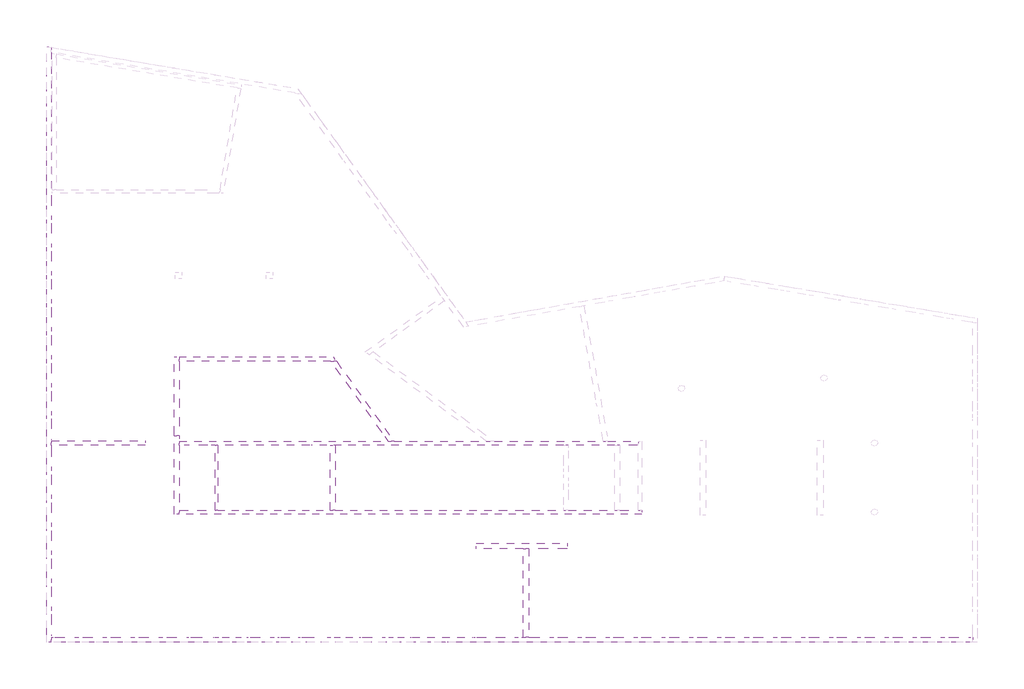
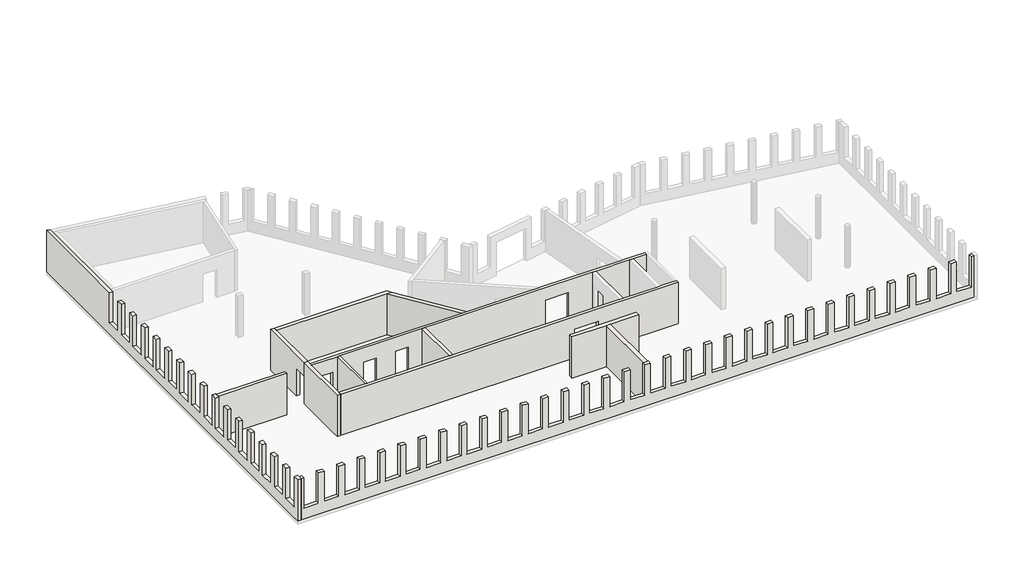
# One storey, part 1 of 2: 13 walls.
"""IFC4 building model written with IfcOpenShell, lengths in millimetres."""

from ifc_helpers import new_model, si_unit, frame, origin, place, context, project, spatial, polyline, outline, extrude, faceted_brep, element, save

model = new_model("IFC4")

# Units and contexts
model_context = context("Model", 3, world=origin())
ifc_project = project(units=[si_unit("LENGTHUNIT", "METRE", prefix="MILLI")], contexts=[model_context])

# Site, building, storey
site = spatial("IfcSite", under=ifc_project)
building = spatial("IfcBuilding", under=site)
storey = spatial("IfcBuildingStorey", under=building, Name="01_UG_OKFB_-4,20", Elevation=-4200.0)

# Walls
placement = place(None, origin())
element("IfcWall", 1, ObjectType="5dki Lochfassade 26cm C30/37", at=placement, inside=storey, context=model_context, shape_type="Brep", body=[
    faceted_brep([(130.0010047, 22777.9895381, 710.0), (130.0010047, 22777.9895381, 3060.0), (130.0010047, 22357.0124158, 3060.0), (130.0010047, 22357.0124158, 710.0), (130.0010047, 21277.0124158, 710.0), (130.0010047, 21277.0124158, 3060.0), (130.0010047, 20857.0124158, 3060.0), (130.0010047, 20857.0124158, 710.0), (130.0010047, 19777.0124158, 710.0), (130.0010047, 19777.0124158, 3060.0), (130.0010047, 19357.0124158, 3060.0), (130.0010047, 19357.0124158, 710.0), (130.0010047, 18277.0124158, 710.0), (130.0010047, 18277.0124158, 3060.0), (130.0010047, 17857.0124158, 3060.0), (130.0010047, 17857.0124158, 710.0), (130.0010047, 16777.0124158, 710.0), (130.0010047, 16777.0124158, 3060.0), (130.0010047, 16357.0124158, 3060.0), (130.0010047, 16357.0124158, 710.0), (130.0010047, 15277.0124158, 710.0), (130.0010047, 15277.0124158, 3060.0), (130.0010047, 14857.0124158, 3060.0), (130.0010047, 14857.0124158, 710.0), (130.0010047, 13777.0124158, 710.0), (130.0010047, 13777.0124158, 3060.0), (130.0010047, 13357.0124158, 3060.0), (130.0010047, 13357.0124158, 710.0), (130.0010047, 12277.0124158, 710.0), (130.0010047, 12277.0124158, 3060.0), (130.0010047, 11857.0124158, 3060.0), (130.0010047, 11857.0124158, 710.0), (130.0010047, 10777.0124158, 710.0), (130.0010047, 10777.0124158, 3060.0), (130.0010047, 10692.0124295, 3060.0), (130.0010047, 10442.0124295, 3060.0), (130.0010047, 10357.0124158, 3060.0), (130.0010047, 10357.0124158, 710.0), (130.0010047, 9277.0124158, 710.0), (130.0010047, 9277.0124158, 3060.0), (130.0010047, 8857.0124158, 3060.0), (130.0010047, 8857.0124158, 710.0), (130.0010047, 7777.0124158, 710.0), (130.0010047, 7777.0124158, 3060.0), (130.0010047, 7357.0124158, 3060.0), (130.0010047, 7357.0124158, 710.0), (130.0010047, 6277.0124158, 710.0), (130.0010047, 6277.0124158, 3060.0), (130.0010047, 5857.0124158, 3060.0), (130.0010047, 5857.0124158, 710.0), (130.0010047, 4777.0124158, 710.0), (130.0010047, 4777.0124158, 3060.0), (130.0010047, 4357.0124158, 3060.0), (130.0010047, 4357.0124158, 710.0), (130.0010047, 3277.0124158, 710.0), (130.0010047, 3277.0124158, 3060.0), (130.0010047, 2857.0124158, 3060.0), (130.0010047, 2857.0124158, 710.0), (130.0010047, 1777.0124158, 710.0), (130.0010047, 1777.0124158, 3060.0), (130.0010047, 1357.0124158, 3060.0), (130.0010047, 1357.0124158, 710.0), (130.0010047, 277.0124158, 710.0), (130.0010047, 277.0124158, 3060.0), (130.0010047, 130.000972, 3060.0), (130.0010047, -129.999028, 3060.0), (130.0010047, -129.999028, -150.0), (130.0010047, 130.000972, -150.0), (130.0010047, 10442.0124295, -150.0), (130.0010047, 10692.0124295, -150.0), (130.0010047, 31548.6978518, -150.0), (130.0010047, 31812.2980067, -150.0), (130.0010047, 31812.2980067, 3060.0), (130.0010047, 31548.6978518, 3060.0), (130.0010047, 23857.9895381, 3060.0), (130.0010047, 23857.9895381, 710.0), (-129.9989953, 22357.0124158, 3060.0), (-129.9989953, 22777.9895381, 3060.0), (-129.9989953, 22777.9895381, 710.0), (-129.9989953, 23857.9895381, 710.0), (-129.9989953, 23857.9895381, 3060.0), (-129.9989953, 31855.7150729, 3060.0), (-129.9989953, 31855.7150729, -150.0), (-129.9989953, -129.9990284, -150.0), (-129.9989953, -129.9990284, 3060.0), (-129.9989953, 277.0124158, 3060.0), (-129.9989953, 277.0124158, 710.0), (-129.9989953, 1357.0124158, 710.0), (-129.9989953, 1357.0124158, 3060.0), (-129.9989953, 1777.0124158, 3060.0), (-129.9989953, 1777.0124158, 710.0), (-129.9989953, 2857.0124158, 710.0), (-129.9989953, 2857.0124158, 3060.0), (-129.9989953, 3277.0124158, 3060.0), (-129.9989953, 3277.0124158, 710.0), (-129.9989953, 4357.0124158, 710.0), (-129.9989953, 4357.0124158, 3060.0), (-129.9989953, 4777.0124158, 3060.0), (-129.9989953, 4777.0124158, 710.0), (-129.9989953, 5857.0124158, 710.0), (-129.9989953, 5857.0124158, 3060.0), (-129.9989953, 6277.0124158, 3060.0), (-129.9989953, 6277.0124158, 710.0), (-129.9989953, 7357.0124158, 710.0), (-129.9989953, 7357.0124158, 3060.0), (-129.9989953, 7777.0124158, 3060.0), (-129.9989953, 7777.0124158, 710.0), (-129.9989953, 8857.0124158, 710.0), (-129.9989953, 8857.0124158, 3060.0), (-129.9989953, 9277.0124158, 3060.0), (-129.9989953, 9277.0124158, 710.0), (-129.9989953, 10357.0124158, 710.0), (-129.9989953, 10357.0124158, 3060.0), (-129.9989953, 10777.0124158, 3060.0), (-129.9989953, 10777.0124158, 710.0), (-129.9989953, 11857.0124158, 710.0), (-129.9989953, 11857.0124158, 3060.0), (-129.9989953, 12277.0124158, 3060.0), (-129.9989953, 12277.0124158, 710.0), (-129.9989953, 13357.0124158, 710.0), (-129.9989953, 13357.0124158, 3060.0), (-129.9989953, 13777.0124158, 3060.0), (-129.9989953, 13777.0124158, 710.0), (-129.9989953, 14857.0124158, 710.0), (-129.9989953, 14857.0124158, 3060.0), (-129.9989953, 15277.0124158, 3060.0), (-129.9989953, 15277.0124158, 710.0), (-129.9989953, 16357.0124158, 710.0), (-129.9989953, 16357.0124158, 3060.0), (-129.9989953, 16777.0124158, 3060.0), (-129.9989953, 16777.0124158, 710.0), (-129.9989953, 17857.0124158, 710.0), (-129.9989953, 17857.0124158, 3060.0), (-129.9989953, 18277.0124158, 3060.0), (-129.9989953, 18277.0124158, 710.0), (-129.9989953, 19357.0124158, 710.0), (-129.9989953, 19357.0124158, 3060.0), (-129.9989953, 19777.0124158, 3060.0), (-129.9989953, 19777.0124158, 710.0), (-129.9989953, 20857.0124158, 710.0), (-129.9989953, 20857.0124158, 3060.0), (-129.9989953, 21277.0124158, 3060.0), (-129.9989953, 21277.0124158, 710.0), (-129.9989953, 22357.0124158, 710.0)], [[[0, 1, 2, 3, 4, 5, 6, 7, 8, 9, 10, 11, 12, 13, 14, 15, 16, 17, 18, 19, 20, 21, 22, 23, 24, 25, 26, 27, 28, 29, 30, 31, 32, 33, 34, 35, 36, 37, 38, 39, 40, 41, 42, 43, 44, 45, 46, 47, 48, 49, 50, 51, 52, 53, 54, 55, 56, 57, 58, 59, 60, 61, 62, 63, 64, 65, 66, 67, 68, 69, 70, 71, 72, 73, 74, 75]], [[76, 77, 78, 79, 80, 81, 82, 83, 84, 85, 86, 87, 88, 89, 90, 91, 92, 93, 94, 95, 96, 97, 98, 99, 100, 101, 102, 103, 104, 105, 106, 107, 108, 109, 110, 111, 112, 113, 114, 115, 116, 117, 118, 119, 120, 121, 122, 123, 124, 125, 126, 127, 128, 129, 130, 131, 132, 133, 134, 135, 136, 137, 138, 139, 140, 141, 142, 143]], [[71, 70, 69, 68, 67, 66, 83, 82]], [[84, 65, 64, 63, 85]], [[60, 59, 89, 88]], [[56, 55, 93, 92]], [[52, 51, 97, 96]], [[48, 47, 101, 100]], [[44, 43, 105, 104]], [[40, 39, 109, 108]], [[36, 35, 34, 33, 113, 112]], [[30, 29, 117, 116]], [[26, 25, 121, 120]], [[22, 21, 125, 124]], [[18, 17, 129, 128]], [[14, 13, 133, 132]], [[10, 9, 137, 136]], [[6, 5, 141, 140]], [[2, 1, 77, 76]], [[74, 73, 72, 81, 80]], [[72, 71, 82, 81]], [[66, 65, 84, 83]], [[87, 61, 60, 88]], [[62, 86, 85, 63]], [[61, 87, 86, 62]], [[92, 91, 57, 56]], [[90, 89, 59, 58]], [[91, 90, 58, 57]], [[96, 95, 53, 52]], [[94, 93, 55, 54]], [[95, 94, 54, 53]], [[100, 99, 49, 48]], [[98, 97, 51, 50]], [[99, 98, 50, 49]], [[104, 103, 45, 44]], [[102, 101, 47, 46]], [[103, 102, 46, 45]], [[108, 107, 41, 40]], [[106, 105, 43, 42]], [[107, 106, 42, 41]], [[112, 111, 37, 36]], [[110, 109, 39, 38]], [[111, 110, 38, 37]], [[116, 115, 31, 30]], [[114, 113, 33, 32]], [[115, 114, 32, 31]], [[120, 119, 27, 26]], [[118, 117, 29, 28]], [[119, 118, 28, 27]], [[124, 123, 23, 22]], [[122, 121, 25, 24]], [[123, 122, 24, 23]], [[128, 127, 19, 18]], [[126, 125, 21, 20]], [[127, 126, 20, 19]], [[132, 131, 15, 14]], [[130, 129, 17, 16]], [[131, 130, 16, 15]], [[136, 135, 11, 10]], [[134, 133, 13, 12]], [[135, 134, 12, 11]], [[140, 139, 7, 6]], [[138, 137, 9, 8]], [[139, 138, 8, 7]], [[76, 143, 3, 2]], [[142, 141, 5, 4]], [[143, 142, 4, 3]], [[80, 79, 75, 74]], [[78, 77, 1, 0]], [[79, 78, 0, 75]]]),
])
element("IfcWall", 2, ObjectType="5dki Lochfassade 26cm C30/37", at=placement, inside=storey, context=model_context, shape_type="Brep", body=[
    faceted_brep([(49396.9999991, 130.0010483, 710.0), (49396.9999991, 130.0010483, 3060.0), (49603.9991101, 130.0010486, 3060.0), (49603.9991101, 130.0010486, -150.0), (25766.9999915, 130.0010117, -150.0), (25466.9999915, 130.0010113, -150.0), (130.0010047, 130.000972, -150.0), (130.0010047, 130.000972, 3060.0), (317.0000012, 130.0009723, 3060.0), (316.999997, 130.0009723, 710.0), (1397.0000012, 130.000974, 710.0), (1397.0000069, 130.000974, 3060.0), (1816.9999991, 130.0009747, 3060.0), (1817.0000028, 130.0009747, 710.0), (2896.9999991, 130.0009763, 710.0), (2897.0000017, 130.0009763, 3060.0), (3316.9999991, 130.000977, 3060.0), (3316.9999977, 130.000977, 710.0), (4396.9999991, 130.0009787, 710.0), (4396.9999966, 130.0009787, 3060.0), (4816.9999991, 130.0009793, 3060.0), (4816.9999991, 130.0009793, 710.0), (5896.9999991, 130.000981, 710.0), (5896.9999991, 130.000981, 3060.0), (6316.9999991, 130.0009816, 3060.0), (6316.9999991, 130.0009816, 710.0), (7396.9999991, 130.0009833, 710.0), (7396.9999991, 130.0009833, 3060.0), (7816.9999991, 130.0009839, 3060.0), (7816.9999991, 130.0009839, 710.0), (8896.9999991, 130.0009856, 710.0), (8896.9999991, 130.0009856, 3060.0), (9316.9999991, 130.0009863, 3060.0), (9316.9999991, 130.0009863, 710.0), (10396.9999991, 130.0009879, 710.0), (10396.9999991, 130.0009879, 3060.0), (10816.9999991, 130.0009886, 3060.0), (10816.9999991, 130.0009886, 710.0), (11896.9999991, 130.0009903, 710.0), (11896.9999991, 130.0009903, 3060.0), (12316.9999991, 130.0009909, 3060.0), (12316.9999991, 130.0009909, 710.0), (13396.9999991, 130.0009926, 710.0), (13396.9999991, 130.0009926, 3060.0), (13816.9999991, 130.0009932, 3060.0), (13816.9999991, 130.0009932, 710.0), (14896.9999991, 130.0009949, 710.0), (14896.9999991, 130.0009949, 3060.0), (15316.9999991, 130.0009956, 3060.0), (15316.9999991, 130.0009956, 710.0), (16396.9999991, 130.0009972, 710.0), (16396.9999991, 130.0009972, 3060.0), (16816.9999991, 130.0009979, 3060.0), (16816.9999991, 130.0009979, 710.0), (17896.9999991, 130.0009996, 710.0), (17896.9999991, 130.0009996, 3060.0), (18316.9999991, 130.0010002, 3060.0), (18316.9999991, 130.0010002, 710.0), (19396.9999991, 130.0010019, 710.0), (19396.9999991, 130.0010019, 3060.0), (19816.9999991, 130.0010025, 3060.0), (19816.9999991, 130.0010025, 710.0), (20896.9999991, 130.0010042, 710.0), (20896.9999991, 130.0010042, 3060.0), (21316.9999991, 130.0010048, 3060.0), (21316.9999991, 130.0010048, 710.0), (22396.9999991, 130.0010065, 710.0), (22396.9999991, 130.0010065, 3060.0), (22816.9999991, 130.0010072, 3060.0), (22816.9999991, 130.0010072, 710.0), (23896.9999991, 130.0010088, 710.0), (23896.9999991, 130.0010088, 3060.0), (24316.9999991, 130.0010095, 3060.0), (24316.9999991, 130.0010095, 710.0), (25396.9999991, 130.0010112, 710.0), (25396.9999991, 130.0010112, 3060.0), (25466.9999915, 130.0010113, 3060.0), (25766.9999915, 130.0010117, 3060.0), (25816.9999991, 130.0010118, 3060.0), (25816.9999991, 130.0010118, 710.0), (26896.9999991, 130.0010135, 710.0), (26896.9999991, 130.0010135, 3060.0), (27316.9999991, 130.0010141, 3060.0), (27316.9999991, 130.0010141, 710.0), (28396.9999991, 130.0010158, 710.0), (28396.9999991, 130.0010158, 3060.0), (28816.9999991, 130.0010165, 3060.0), (28816.9999991, 130.0010165, 710.0), (29896.9999991, 130.0010181, 710.0), (29896.9999991, 130.0010181, 3060.0), (30316.9999991, 130.0010188, 3060.0), (30316.9999991, 130.0010188, 710.0), (31396.9999991, 130.0010205, 710.0), (31396.9999991, 130.0010205, 3060.0), (31816.9999991, 130.0010211, 3060.0), (31816.9999991, 130.0010211, 710.0), (32896.9999991, 130.0010228, 710.0), (32896.9999991, 130.0010228, 3060.0), (33316.9999991, 130.0010234, 3060.0), (33316.9999991, 130.0010234, 710.0), (34396.9999991, 130.0010251, 710.0), (34396.9999991, 130.0010251, 3060.0), (34816.9999991, 130.0010258, 3060.0), (34816.9999991, 130.0010258, 710.0), (35896.9999991, 130.0010274, 710.0), (35896.9999991, 130.0010274, 3060.0), (36316.9999991, 130.0010281, 3060.0), (36316.9999991, 130.0010281, 710.0), (37396.9999991, 130.0010297, 710.0), (37396.9999991, 130.0010297, 3060.0), (37816.9999991, 130.0010304, 3060.0), (37816.9999991, 130.0010304, 710.0), (38896.9999991, 130.0010321, 710.0), (38896.9999991, 130.0010321, 3060.0), (39316.9999991, 130.0010327, 3060.0), (39316.9999991, 130.0010327, 710.0), (40396.9999991, 130.0010344, 710.0), (40396.9999991, 130.0010344, 3060.0), (40816.9999991, 130.001035, 3060.0), (40816.9999991, 130.001035, 710.0), (41896.9999991, 130.0010367, 710.0), (41896.9999991, 130.0010367, 3060.0), (42316.9999991, 130.0010374, 3060.0), (42316.9999991, 130.0010374, 710.0), (43396.9999991, 130.001039, 710.0), (43396.9999991, 130.001039, 3060.0), (43816.9999991, 130.0010397, 3060.0), (43816.9999991, 130.0010397, 710.0), (44896.9999991, 130.0010414, 710.0), (44896.9999991, 130.0010414, 3060.0), (45316.9999991, 130.001042, 3060.0), (45316.9999991, 130.001042, 710.0), (46396.9999991, 130.0010437, 710.0), (46396.9999991, 130.0010437, 3060.0), (46816.9999991, 130.0010443, 3060.0), (46816.9999991, 130.0010443, 710.0), (47896.9999991, 130.001046, 710.0), (47896.9999991, 130.001046, 3060.0), (48316.9999991, 130.0010467, 3060.0), (48316.9999991, 130.0010467, 710.0), (49603.9991105, -129.9989514, 3060.0), (49396.9999995, -129.9989517, 3060.0), (49396.9999995, -129.9989517, 710.0), (48316.9999995, -129.9989533, 710.0), (48316.9999995, -129.9989533, 3060.0), (47896.9999995, -129.998954, 3060.0), (47896.9999995, -129.998954, 710.0), (46816.9999995, -129.9989557, 710.0), (46816.9999995, -129.9989557, 3060.0), (46396.9999995, -129.9989563, 3060.0), (46396.9999995, -129.9989563, 710.0), (45316.9999995, -129.998958, 710.0), (45316.9999995, -129.998958, 3060.0), (44896.9999995, -129.9989586, 3060.0), (44896.9999995, -129.9989586, 710.0), (43816.9999995, -129.9989603, 710.0), (43816.9999995, -129.9989603, 3060.0), (43396.9999995, -129.998961, 3060.0), (43396.9999995, -129.998961, 710.0), (42316.9999995, -129.9989626, 710.0), (42316.9999995, -129.9989626, 3060.0), (41896.9999995, -129.9989633, 3060.0), (41896.9999995, -129.9989633, 710.0), (40816.9999995, -129.998965, 710.0), (40816.9999995, -129.998965, 3060.0), (40396.9999995, -129.9989656, 3060.0), (40396.9999995, -129.9989656, 710.0), (39316.9999995, -129.9989673, 710.0), (39316.9999995, -129.9989673, 3060.0), (38896.9999995, -129.9989679, 3060.0), (38896.9999995, -129.9989679, 710.0), (37816.9999995, -129.9989696, 710.0), (37816.9999995, -129.9989696, 3060.0), (37396.9999995, -129.9989703, 3060.0), (37396.9999995, -129.9989703, 710.0), (36316.9999995, -129.9989719, 710.0), (36316.9999995, -129.9989719, 3060.0), (35896.9999995, -129.9989726, 3060.0), (35896.9999995, -129.9989726, 710.0), (34816.9999995, -129.9989742, 710.0), (34816.9999995, -129.9989742, 3060.0), (34396.9999995, -129.9989749, 3060.0), (34396.9999995, -129.9989749, 710.0), (33316.9999995, -129.9989766, 710.0), (33316.9999995, -129.9989766, 3060.0), (32896.9999995, -129.9989772, 3060.0), (32896.9999995, -129.9989772, 710.0), (31816.9999995, -129.9989789, 710.0), (31816.9999995, -129.9989789, 3060.0), (31396.9999995, -129.9989795, 3060.0), (31396.9999995, -129.9989795, 710.0), (30316.9999995, -129.9989812, 710.0), (30316.9999995, -129.9989812, 3060.0), (29896.9999995, -129.9989819, 3060.0), (29896.9999995, -129.9989819, 710.0), (28816.9999995, -129.9989835, 710.0), (28816.9999995, -129.9989835, 3060.0), (28396.9999995, -129.9989842, 3060.0), (28396.9999995, -129.9989842, 710.0), (27316.9999995, -129.9989859, 710.0), (27316.9999995, -129.9989859, 3060.0), (26896.9999995, -129.9989865, 3060.0), (26896.9999995, -129.9989865, 710.0), (25816.9999995, -129.9989882, 710.0), (25816.9999995, -129.9989882, 3060.0), (25396.9999995, -129.9989888, 3060.0), (25396.9999995, -129.9989888, 710.0), (24316.9999995, -129.9989905, 710.0), (24316.9999995, -129.9989905, 3060.0), (23896.9999995, -129.9989912, 3060.0), (23896.9999995, -129.9989912, 710.0), (22816.9999995, -129.9989928, 710.0), (22816.9999995, -129.9989928, 3060.0), (22396.9999995, -129.9989935, 3060.0), (22396.9999995, -129.9989935, 710.0), (21316.9999995, -129.9989952, 710.0), (21316.9999995, -129.9989952, 3060.0), (20896.9999995, -129.9989958, 3060.0), (20896.9999995, -129.9989958, 710.0), (19816.9999995, -129.9989975, 710.0), (19816.9999995, -129.9989975, 3060.0), (19396.9999995, -129.9989981, 3060.0), (19396.9999995, -129.9989981, 710.0), (18316.9999995, -129.9989998, 710.0), (18316.9999995, -129.9989998, 3060.0), (17896.9999995, -129.9990004, 3060.0), (17896.9999995, -129.9990004, 710.0), (16816.9999995, -129.9990021, 710.0), (16816.9999995, -129.9990021, 3060.0), (16396.9999995, -129.9990028, 3060.0), (16396.9999995, -129.9990028, 710.0), (15316.9999995, -129.9990044, 710.0), (15316.9999995, -129.9990044, 3060.0), (14896.9999995, -129.9990051, 3060.0), (14896.9999995, -129.9990051, 710.0), (13816.9999995, -129.9990068, 710.0), (13816.9999995, -129.9990068, 3060.0), (13396.9999995, -129.9990074, 3060.0), (13396.9999995, -129.9990074, 710.0), (12316.9999995, -129.9990091, 710.0), (12316.9999995, -129.9990091, 3060.0), (11896.9999995, -129.9990097, 3060.0), (11896.9999995, -129.9990097, 710.0), (10816.9999995, -129.9990114, 710.0), (10816.9999995, -129.9990114, 3060.0), (10396.9999995, -129.9990121, 3060.0), (10396.9999995, -129.9990121, 710.0), (9316.9999995, -129.9990137, 710.0), (9316.9999995, -129.9990137, 3060.0), (8896.9999995, -129.9990144, 3060.0), (8896.9999995, -129.9990144, 710.0), (7816.9999995, -129.9990161, 710.0), (7816.9999995, -129.9990161, 3060.0), (7396.9999995, -129.9990167, 3060.0), (7396.9999995, -129.9990167, 710.0), (6316.9999995, -129.9990184, 710.0), (6316.9999995, -129.9990184, 3060.0), (5896.9999995, -129.999019, 3060.0), (5896.9999995, -129.999019, 710.0), (4816.9999995, -129.9990207, 710.0), (4816.9999995, -129.9990207, 3060.0), (4396.9999995, -129.9990213, 3060.0), (4396.9999966, -129.9990213, 710.0), (3316.9999995, -129.999023, 710.0), (3316.9999977, -129.999023, 3060.0), (2896.9999995, -129.9990237, 3060.0), (2897.0000017, -129.9990237, 710.0), (1816.9999995, -129.9990253, 710.0), (1817.0000028, -129.9990253, 3060.0), (1397.0000016, -129.999026, 3060.0), (1397.0000069, -129.999026, 710.0), (317.0000016, -129.9990277, 710.0), (316.999997, -129.9990277, 3060.0), (130.0010047, -129.999028, 3060.0), (130.0010047, -129.999028, -150.0), (49603.9991105, -129.9989514, -150.0)], [[[0, 1, 2, 3, 4, 5, 6, 7, 8, 9, 10, 11, 12, 13, 14, 15, 16, 17, 18, 19, 20, 21, 22, 23, 24, 25, 26, 27, 28, 29, 30, 31, 32, 33, 34, 35, 36, 37, 38, 39, 40, 41, 42, 43, 44, 45, 46, 47, 48, 49, 50, 51, 52, 53, 54, 55, 56, 57, 58, 59, 60, 61, 62, 63, 64, 65, 66, 67, 68, 69, 70, 71, 72, 73, 74, 75, 76, 77, 78, 79, 80, 81, 82, 83, 84, 85, 86, 87, 88, 89, 90, 91, 92, 93, 94, 95, 96, 97, 98, 99, 100, 101, 102, 103, 104, 105, 106, 107, 108, 109, 110, 111, 112, 113, 114, 115, 116, 117, 118, 119, 120, 121, 122, 123, 124, 125, 126, 127, 128, 129, 130, 131, 132, 133, 134, 135, 136, 137, 138, 139]], [[140, 141, 142, 143, 144, 145, 146, 147, 148, 149, 150, 151, 152, 153, 154, 155, 156, 157, 158, 159, 160, 161, 162, 163, 164, 165, 166, 167, 168, 169, 170, 171, 172, 173, 174, 175, 176, 177, 178, 179, 180, 181, 182, 183, 184, 185, 186, 187, 188, 189, 190, 191, 192, 193, 194, 195, 196, 197, 198, 199, 200, 201, 202, 203, 204, 205, 206, 207, 208, 209, 210, 211, 212, 213, 214, 215, 216, 217, 218, 219, 220, 221, 222, 223, 224, 225, 226, 227, 228, 229, 230, 231, 232, 233, 234, 235, 236, 237, 238, 239, 240, 241, 242, 243, 244, 245, 246, 247, 248, 249, 250, 251, 252, 253, 254, 255, 256, 257, 258, 259, 260, 261, 262, 263, 264, 265, 266, 267, 268, 269, 270, 271, 272, 273, 274, 275]], [[6, 5, 4, 3, 275, 274]], [[7, 273, 272, 8]], [[15, 265, 264, 16]], [[268, 12, 11, 269]], [[261, 260, 20, 19]], [[257, 256, 24, 23]], [[253, 252, 28, 27]], [[249, 248, 32, 31]], [[245, 244, 36, 35]], [[241, 240, 40, 39]], [[237, 236, 44, 43]], [[233, 232, 48, 47]], [[229, 228, 52, 51]], [[225, 224, 56, 55]], [[221, 220, 60, 59]], [[217, 216, 64, 63]], [[213, 212, 68, 67]], [[209, 208, 72, 71]], [[205, 204, 78, 77, 76, 75]], [[201, 200, 82, 81]], [[197, 196, 86, 85]], [[193, 192, 90, 89]], [[189, 188, 94, 93]], [[185, 184, 98, 97]], [[181, 180, 102, 101]], [[177, 176, 106, 105]], [[173, 172, 110, 109]], [[169, 168, 114, 113]], [[165, 164, 118, 117]], [[161, 160, 122, 121]], [[157, 156, 126, 125]], [[153, 152, 130, 129]], [[149, 148, 134, 133]], [[138, 137, 145, 144]], [[2, 1, 141, 140]], [[7, 6, 274, 273]], [[3, 2, 140, 275]], [[10, 270, 269, 11]], [[271, 9, 8, 272]], [[270, 10, 9, 271]], [[14, 266, 265, 15]], [[267, 13, 12, 268]], [[266, 14, 13, 267]], [[18, 262, 261, 19]], [[263, 17, 16, 264]], [[262, 18, 17, 263]], [[23, 22, 258, 257]], [[21, 20, 260, 259]], [[22, 21, 259, 258]], [[27, 26, 254, 253]], [[25, 24, 256, 255]], [[26, 25, 255, 254]], [[31, 30, 250, 249]], [[29, 28, 252, 251]], [[30, 29, 251, 250]], [[35, 34, 246, 245]], [[33, 32, 248, 247]], [[34, 33, 247, 246]], [[39, 38, 242, 241]], [[37, 36, 244, 243]], [[38, 37, 243, 242]], [[43, 42, 238, 237]], [[41, 40, 240, 239]], [[42, 41, 239, 238]], [[47, 46, 234, 233]], [[45, 44, 236, 235]], [[46, 45, 235, 234]], [[51, 50, 230, 229]], [[49, 48, 232, 231]], [[50, 49, 231, 230]], [[55, 54, 226, 225]], [[53, 52, 228, 227]], [[54, 53, 227, 226]], [[59, 58, 222, 221]], [[57, 56, 224, 223]], [[58, 57, 223, 222]], [[63, 62, 218, 217]], [[61, 60, 220, 219]], [[62, 61, 219, 218]], [[67, 66, 214, 213]], [[65, 64, 216, 215]], [[66, 65, 215, 214]], [[71, 70, 210, 209]], [[69, 68, 212, 211]], [[70, 69, 211, 210]], [[75, 74, 206, 205]], [[73, 72, 208, 207]], [[74, 73, 207, 206]], [[81, 80, 202, 201]], [[79, 78, 204, 203]], [[80, 79, 203, 202]], [[85, 84, 198, 197]], [[83, 82, 200, 199]], [[84, 83, 199, 198]], [[89, 88, 194, 193]], [[87, 86, 196, 195]], [[88, 87, 195, 194]], [[93, 92, 190, 189]], [[91, 90, 192, 191]], [[92, 91, 191, 190]], [[97, 96, 186, 185]], [[95, 94, 188, 187]], [[96, 95, 187, 186]], [[101, 100, 182, 181]], [[99, 98, 184, 183]], [[100, 99, 183, 182]], [[105, 104, 178, 177]], [[103, 102, 180, 179]], [[104, 103, 179, 178]], [[109, 108, 174, 173]], [[107, 106, 176, 175]], [[108, 107, 175, 174]], [[113, 112, 170, 169]], [[111, 110, 172, 171]], [[112, 111, 171, 170]], [[117, 116, 166, 165]], [[115, 114, 168, 167]], [[116, 115, 167, 166]], [[121, 120, 162, 161]], [[119, 118, 164, 163]], [[120, 119, 163, 162]], [[125, 124, 158, 157]], [[123, 122, 160, 159]], [[124, 123, 159, 158]], [[129, 128, 154, 153]], [[127, 126, 156, 155]], [[128, 127, 155, 154]], [[133, 132, 150, 149]], [[131, 130, 152, 151]], [[132, 131, 151, 150]], [[137, 136, 146, 145]], [[135, 134, 148, 147]], [[136, 135, 147, 146]], [[144, 143, 139, 138]], [[142, 141, 1, 0]], [[143, 142, 0, 139]]]),
])
element("IfcWall", 3, ObjectType="5dki STB-Wand Kern 25cm C30/37", at=placement, inside=storey, context=model_context, shape_type="Brep", body=[
    faceted_brep([(6989.9999766, 15192.0124447, 3060.0), (6989.9999766, 14942.0124447, 3060.0), (6989.9999766, 10947.0136187, 3060.0), (6989.9999766, 10947.0136187, 1985.0), (6989.9999766, 11957.013616, 1985.0), (6989.9999766, 11957.013616, -150.0), (6989.9999766, 14942.0124447, -150.0), (6989.9999766, 15192.0124447, -150.0), (6739.9999766, 10947.0136187, 3060.0), (6739.9999766, 15192.0124447, 3060.0), (6739.9999766, 15192.0124447, -150.0), (6739.9999766, 11957.013616, -150.0), (6739.9999766, 11957.013616, 1985.0), (6739.9999766, 10947.0136187, 1985.0)], [[[0, 1, 2, 3, 4, 5, 6, 7]], [[8, 9, 10, 11, 12, 13]], [[10, 7, 6, 5, 11]], [[2, 1, 0, 9, 8]], [[2, 8, 13, 3]], [[0, 7, 10, 9]], [[4, 12, 11, 5]], [[12, 4, 3, 13]]]),
])
element("IfcWall", 4, ObjectType="5dki STB-Wand Kern 25cm C30/37", at=placement, inside=storey, context=model_context, shape_type="Brep", body=[
    faceted_brep([(6989.9999766, 14942.0124447, -150.0), (15141.8279932, 14942.0124447, -150.0), (15449.8792779, 14942.0124447, -150.0), (15449.8792779, 14942.0124447, 3060.0), (15141.8279932, 14942.0124447, 3060.0), (6989.9999766, 14942.0124447, 3060.0), (6989.9999766, 15192.0124447, -150.0), (6989.9999766, 15192.0124447, 3060.0), (15269.8915173, 15192.0124447, 3060.0), (15269.8915173, 15192.0124447, -150.0)], [[[0, 1, 2, 3, 4, 5]], [[6, 7, 8, 9]], [[2, 1, 0, 6, 9]], [[5, 4, 3, 8, 7]], [[0, 5, 7, 6]], [[3, 2, 9, 8]]]),
])
element("IfcWall", 5, ObjectType="5dki STB-Wand Kern 25cm C30/37", at=placement, inside=storey, context=model_context, shape_type="Brep", body=[
    faceted_brep([(18223.2182524, 10662.0127257, 3060.0), (15141.8279932, 14942.0124447, 3060.0), (15141.8279932, 14942.0124447, -150.0), (17305.3310134, 11936.9428041, -150.0), (17305.3310134, 11936.9428041, 1985.0), (17895.4523577, 11117.2740911, 1985.0), (17895.4523577, 11117.2740911, -150.0), (18223.2182524, 10662.0127257, -150.0), (15449.8792779, 14942.0124447, 3060.0), (18531.2695366, 10662.0127262, 3060.0), (18531.2695366, 10662.0127262, -150.0), (18098.340653, 11263.3437308, -150.0), (18098.340653, 11263.3437308, 1985.0), (17508.2193087, 12083.0124438, 1985.0), (17508.2193087, 12083.0124438, -150.0), (15449.8792779, 14942.0124447, -150.0)], [[[0, 1, 2, 3, 4, 5, 6, 7]], [[8, 9, 10, 11, 12, 13, 14, 15]], [[2, 15, 14, 3]], [[10, 7, 6, 11]], [[1, 0, 9, 8]], [[2, 1, 8, 15]], [[0, 7, 10, 9]], [[13, 4, 3, 14]], [[4, 13, 12, 5]], [[5, 12, 11, 6]]]),
])
element("IfcWall", 6, ObjectType="5dki STB-Wand Kern 25cm C30/37", at=placement, inside=storey, context=model_context, shape_type="Brep", body=[
    faceted_brep([(6739.9995723, 10947.0136187, -150.0), (6739.9995723, 6740.0000204, -150.0), (6739.9995723, 6740.0000204, 3060.0), (6739.9995723, 10947.0136187, 3060.0), (6989.9995723, 10947.0136187, -150.0), (6989.9995723, 10947.0136187, 3060.0), (6989.9995723, 10662.0127052, 3060.0), (6989.9995723, 10442.0127052, 3060.0), (6989.9995723, 6960.0000208, 3060.0), (6989.9995723, 6740.0000208, 3060.0), (6989.9995723, 6740.0000208, -150.0), (6989.9995723, 6960.0000208, -150.0), (6989.9995723, 10442.0127052, -150.0), (6989.9995723, 10662.0127052, -150.0)], [[[0, 1, 2, 3]], [[4, 5, 6, 7, 8, 9, 10, 11, 12, 13]], [[1, 0, 4, 13, 12, 11, 10]], [[3, 2, 9, 8, 7, 6, 5]], [[0, 3, 5, 4]], [[2, 1, 10, 9]]]),
])
element("IfcWall", 7, ObjectType="5dki STB-Wand Kern 22cm C30/37", at=placement, inside=storey, context=model_context, shape_type="Brep", body=[
    faceted_brep([(31841.999935, 6740.0000516, 3060.0), (6989.9995723, 6740.0000208, 3060.0), (6989.9995723, 6740.0000208, -150.0), (24166.9999591, 6740.0000421, -150.0), (24166.999888, 6740.0000421, 2110.0), (25926.9999591, 6740.0000443, 2110.0), (25927.000338, 6740.0000443, -150.0), (31841.999935, 6740.0000516, -150.0), (6989.9995723, 6960.0000208, 3060.0), (8916.9999886, 6960.0000232, 3060.0), (9066.9999886, 6960.0000233, 3060.0), (15117.0008797, 6960.0000309, 3060.0), (15367.0008797, 6960.0000312, 3060.0), (27641.9999886, 6960.0000464, 3060.0), (27891.9999886, 6960.0000467, 3060.0), (30391.9999891, 6960.0000498, 3060.0), (30641.9999891, 6960.0000501, 3060.0), (31641.9999382, 6960.0000514, 3060.0), (31841.9999382, 6960.0000516, 3060.0), (31841.9999382, 6960.0000516, -150.0), (31641.9999382, 6960.0000514, -150.0), (30641.9999891, 6960.0000501, -150.0), (30391.9999891, 6960.0000498, -150.0), (27891.9999886, 6960.0000467, -150.0), (27641.9999886, 6960.0000464, -150.0), (25926.9999588, 6960.0000443, -150.0), (25927.000338, 6960.0000443, 2110.0), (24166.9999588, 6960.0000421, 2110.0), (24166.999888, 6960.0000421, -150.0), (15367.0008797, 6960.0000312, -150.0), (15117.0008797, 6960.0000309, -150.0), (9066.9999886, 6960.0000233, -150.0), (8916.9999886, 6960.0000232, -150.0), (6989.9995723, 6960.0000208, -150.0)], [[[0, 1, 2, 3, 4, 5, 6, 7]], [[8, 9, 10, 11, 12, 13, 14, 15, 16, 17, 18, 19, 20, 21, 22, 23, 24, 25, 26, 27, 28, 29, 30, 31, 32, 33]], [[2, 33, 32, 31, 30, 29, 28, 3]], [[19, 7, 6, 25, 24, 23, 22, 21, 20]], [[1, 0, 18, 17, 16, 15, 14, 13, 12, 11, 10, 9, 8]], [[2, 1, 8, 33]], [[0, 7, 19, 18]], [[5, 26, 25, 6]], [[26, 5, 4, 27]], [[27, 4, 3, 28]]]),
])
element("IfcWall", 8, ObjectType="5dki STB-Wand Kern 22cm C30/37", at=placement, inside=storey, context=model_context, shape_type="Brep", body=[
    faceted_brep([(6989.9995723, 10662.0127052, 3060.0), (18223.2182524, 10662.0127257, 3060.0), (18531.2695366, 10662.0127262, 3060.0), (23491.8764947, 10662.0127353, 3060.0), (23912.428752, 10662.0127361, 3060.0), (29768.165987, 10662.0127467, 3060.0), (30022.0739196, 10662.0127472, 3060.0), (31641.9999912, 10662.0127502, 3060.0), (31641.9999912, 10662.0127502, -150.0), (30022.0739196, 10662.0127472, -150.0), (29768.165987, 10662.0127467, -150.0), (25926.999945, 10662.0127397, -150.0), (25927.0000254, 10662.0127397, 2110.0), (24166.999945, 10662.0127365, 2110.0), (24166.9998144, 10662.0127365, -150.0), (23912.428752, 10662.0127361, -150.0), (23491.8764947, 10662.0127353, -150.0), (18531.2695366, 10662.0127262, -150.0), (18223.2182524, 10662.0127257, -150.0), (14152.0004935, 10662.0127182, -150.0), (14152.0007698, 10662.0127182, 1985.0), (13142.0004935, 10662.0127164, 1985.0), (13142.0009721, 10662.0127164, -150.0), (11796.9999806, 10662.0127139, -150.0), (11796.9997327, 10662.0127139, 1985.0), (10786.9999806, 10662.0127121, 1985.0), (10786.999935, 10662.0127121, -150.0), (8540.0010342, 10662.012708, -150.0), (8540.000485, 10662.012708, 1985.0), (7530.0010342, 10662.0127061, 1985.0), (7530.0006873, 10662.0127061, -150.0), (6989.9995723, 10662.0127052, -150.0), (31641.9999881, 10442.0127502, 3060.0), (30641.9999891, 10442.0127483, 3060.0), (30391.9999891, 10442.0127479, 3060.0), (27891.9999829, 10442.0127433, 3060.0), (27641.9999829, 10442.0127429, 3060.0), (9066.9999886, 10442.0127089, 3060.0), (8916.9999886, 10442.0127087, 3060.0), (6989.9995723, 10442.0127052, 3060.0), (6989.9995723, 10442.0127052, -150.0), (7530.0010346, 10442.0127061, -150.0), (7530.0006873, 10442.0127061, 1985.0), (8540.0010346, 10442.012708, 1985.0), (8540.000485, 10442.012708, -150.0), (8916.9999886, 10442.0127087, -150.0), (9066.9999886, 10442.0127089, -150.0), (10786.999981, 10442.0127121, -150.0), (10786.999935, 10442.0127121, 1985.0), (11796.999981, 10442.0127139, 1985.0), (11796.9997327, 10442.0127139, -150.0), (13142.0004939, 10442.0127164, -150.0), (13142.0009721, 10442.0127164, 1985.0), (14152.0004939, 10442.0127182, 1985.0), (14152.0007698, 10442.0127182, -150.0), (24166.9999454, 10442.0127365, -150.0), (24166.9998144, 10442.0127365, 2110.0), (25926.9999454, 10442.0127397, 2110.0), (25927.0000254, 10442.0127397, -150.0), (27641.9999829, 10442.0127429, -150.0), (27891.9999829, 10442.0127433, -150.0), (30391.9999891, 10442.0127479, -150.0), (30641.9999891, 10442.0127483, -150.0), (31641.9999881, 10442.0127502, -150.0)], [[[0, 1, 2, 3, 4, 5, 6, 7, 8, 9, 10, 11, 12, 13, 14, 15, 16, 17, 18, 19, 20, 21, 22, 23, 24, 25, 26, 27, 28, 29, 30, 31]], [[32, 33, 34, 35, 36, 37, 38, 39, 40, 41, 42, 43, 44, 45, 46, 47, 48, 49, 50, 51, 52, 53, 54, 55, 56, 57, 58, 59, 60, 61, 62, 63]], [[40, 31, 30, 41]], [[8, 63, 62, 61, 60, 59, 58, 11, 10, 9]], [[14, 55, 54, 19, 18, 17, 16, 15]], [[26, 47, 46, 45, 44, 27]], [[50, 23, 22, 51]], [[7, 6, 5, 4, 3, 2, 1, 0, 39, 38, 37, 36, 35, 34, 33, 32]], [[0, 31, 40, 39]], [[8, 7, 32, 63]], [[57, 12, 11, 58]], [[12, 57, 56, 13]], [[13, 56, 55, 14]], [[25, 48, 47, 26]], [[48, 25, 24, 49]], [[49, 24, 23, 50]], [[21, 52, 51, 22]], [[52, 21, 20, 53]], [[53, 20, 19, 54]], [[29, 42, 41, 30]], [[42, 29, 28, 43]], [[43, 28, 27, 44]]]),
])
element("IfcWall", 9, ObjectType="5dki STB-Wand Kern 25cm C30/37", at=placement, inside=storey, context=model_context, shape_type="SweptSolid", body=[
    extrude(outline(polyline([(15117.0008797, 6960.0000309), (15117.0008797, 10442.0127204), (15367.0008797, 10442.0127204), (15367.0008797, 6960.0000312), (15117.0008797, 6960.0000309)])), frame((0.0, 0.0, -150.0), z_axis=(0.0, 0.0, 1.0), x_axis=(1.0, 0.0, 0.0)), (0.0, 0.0, 1.0), 3210.0),
])
element("IfcWall", 10, ObjectType="5dki STB-Wand Kern 15cm C30/37", at=placement, inside=storey, context=model_context, shape_type="SweptSolid", body=[
    extrude(outline(polyline([(8916.9999886, 6960.0000232), (8916.9999886, 10442.0127087), (9066.9999886, 10442.0127089), (9066.9999886, 6960.0000233), (8916.9999886, 6960.0000232)])), frame((0.0, 0.0, -150.0), z_axis=(0.0, 0.0, 1.0), x_axis=(1.0, 0.0, 0.0)), (0.0, 0.0, 1.0), 3210.0),
])
element("IfcWall", 11, ObjectType="5dki STB-Wand 25cm C30/37", at=placement, inside=storey, context=model_context, shape_type="SweptSolid", body=[
    extrude(outline(polyline([(130.0010047, 10692.0124295), (5179.9999831, 10692.0124295), (5179.9999831, 10442.0124295), (130.0010047, 10442.0124295), (130.0010047, 10692.0124295)])), frame((0.0, 0.0, -150.0), z_axis=(0.0, 0.0, 1.0), x_axis=(1.0, 0.0, 0.0)), (0.0, 0.0, 1.0), 3210.0),
])
element("IfcWall", 12, ObjectType="5dki STB-Wand 30cm C30/37", at=placement, inside=storey, context=model_context, shape_type="Brep", body=[
    faceted_brep([(22936.4905033, 4880.0000432, -150.0), (25466.9999915, 4880.0000432, -150.0), (25766.9999915, 4880.0000432, -150.0), (27842.0010332, 4880.0000432, -150.0), (27842.0010332, 4880.0000432, 3060.0), (25766.9999915, 4880.0000432, 3060.0), (25466.9999915, 4880.0000432, 3060.0), (22936.4905033, 4880.0000432, 3060.0), (22936.4905033, 5180.0000432, -150.0), (22936.4905033, 5180.0000432, 3060.0), (27842.0010332, 5180.0000432, 3060.0), (27842.0010332, 5180.0000432, -150.0)], [[[0, 1, 2, 3, 4, 5, 6, 7]], [[8, 9, 10, 11]], [[3, 2, 1, 0, 8, 11]], [[4, 3, 11, 10]], [[7, 6, 5, 4, 10, 9]], [[0, 7, 9, 8]]]),
])
element("IfcWall", 13, ObjectType="5dki STB-Wand 30cm C30/37", at=placement, inside=storey, context=model_context, shape_type="SweptSolid", body=[
    extrude(outline(polyline([(25466.9999915, 130.0010113), (25466.9999915, 4880.0000432), (25766.9999915, 4880.0000432), (25766.9999915, 130.0010117), (25466.9999915, 130.0010113)])), frame((0.0, 0.0, -150.0), z_axis=(0.0, 0.0, 1.0), x_axis=(1.0, 0.0, 0.0)), (0.0, 0.0, 1.0), 3210.0),
])

save(model, "model.ifc")

# Revit data of these elements
# Project information
#   StoreyModel = "<?xml version=\"1.0\" encoding=\"utf-16\"?>\n<StoreyModel xmlns:xsd=\"http://www.w3.org/2001/XMLSchema\" xmlns:xsi=\"http://www.w3.org/2001/XMLSchema-instance\" FormatVersion=\"2013.0.1.0\">\n  <GUID>d780c1b4-dd28-4844-915e-88a2c4b9528b</GUID>\n  <StoreyList />\n  <HelpLevelList />\n  <LastModificationDate>2014-08-27T10:30:40.9523468+02:00</LastModificationDate>\n  <LastModificationAutor>BiesingerMar</LastModificationAutor>\n  <SynchronizedStoreyModelFile />\n  <StandardConfiguration>\n    <Name>5D Standard</Name>\n    <Version>November 2012</Version>\n    <Description>5D-Standardkonfiguration</Description>\n    <LastModificationDate>2012-11-26T14:42:43.0850171+01:00</LastModificationDate>\n    <LastModificationAutor>5D-Administrator</LastModificationAutor>\n    <LevelStandard>\n      <LevelUsageList>\n        <LevelUsage>\n          <ID>0</ID>\n          <Function>Standard</Function>\n          <Name>STRD</Name>\n          <Abbreviation>STRD</Abbreviation>\n        </LevelUsage>\n        <LevelUsage>\n          <ID>1</ID>\n          <Function>Unterkante Rohdecke</Function>\n          <Name>UKRD</Name>\n          <Abbreviation>UKRD</Abbreviation>\n        </LevelUsage>\n        <LevelUsage>\n          <ID>2</ID>\n          <Function>Oberkante Rohdecke</Function>\n          <Name>OKRD</Name>\n          <Abbreviation>OKRD</Abbreviation>\n        </LevelUsage>\n        <LevelUsage>\n          <ID>3</ID>\n          <Function>Oberkante Fertigfußboden</Function>\n          <Name>OKFB</Name>\n          <Abbreviation>OKFB</Abbreviation>\n        </LevelUsage>\n        <LevelUsage>\n          <ID>4</ID>\n          <Function>Unterkante Abgehängter Decke</Function>\n          <Name>UKAD</Name>\n          <Abbreviation>UKAD</Abbreviation>\n        </LevelUsage>\n        <LevelUsage>\n          <ID>5</ID>\n          <Function>Statik</Function>\n          <Name>STAT</Name>\n          <Abbreviation>STAT</Abbreviation>\n        </LevelUsage>\n        <LevelUsage>\n          <ID>100</ID>\n          <Function>Hilfsebene</Function>\n          <Name>HELP</Name>\n          <Abbreviation>HELP</Abbreviation>\n        </LevelUsage>\n        <LevelUsage>\n          <ID>1000</ID>\n          <Function>Oberkante Fundament</Function>\n          <Name>OKFU</Name>\n          <Abbreviation>OKFU</Abbreviation>\n        </LevelUsage>\n        <LevelUsage>\n          <ID>1001</ID>\n          <Function>Unterkante Träger</Function>\n          <Name>UKTR</Name>\n          <Abbreviation>UKTR</Abbreviation>\n        </LevelUsage>\n        <LevelUsage>\n          <ID>1002</ID>\n          <Function>Lift</Function>\n          <Name>LIFT</Name>\n          <Abbreviation>LIFT</Abbreviation>\n        </LevelUsage>\n        <LevelUsage>\n          <ID>1003</ID>\n          <Function>Sockel</Function>\n          <Name>SOCK</Name>\n          <Abbreviation>SOCK</Abbreviation>\n        </LevelUsage>\n        <LevelUsage>\n          <ID>1004</ID>\n          <Function>Wandoberkante</Function>\n          <Name>OKWA</Name>\n          <Abbreviation>OKWA</Abbreviation>\n        </LevelUsage>\n        <LevelUsage>\n          <ID>1005</ID>\n          <Function>Dämmebene</Function>\n          <Name>DAEM</Name>\n          <Abbreviation>DAEM</Abbreviation>\n        </LevelUsage>\n        <LevelUsage>\n          <ID>1006</ID>\n          <Function>OK geneigtes Objekt</Function>\n          <Name>NEIG</Name>\n          <Abbreviation>NEIG</Abbreviation>\n        </LevelUsage>\n        <LevelUsage>\n          <ID>1007</ID>\n          <Function>Außenanlagen</Function>\n          <Name>AUSS</Name>\n          <Abbreviation>AUSS</Abbreviation>\n        </LevelUsage>\n        <LevelUsage>\n          <ID>1008</ID>\n          <Function>Boeschung Oberkante</Function>\n          <Name>BOOK</Name>\n          <Abbreviation>BOOK</Abbreviation>\n        </LevelUsage>\n        <LevelUsage>\n          <ID>1009</ID>\n          <Function>Boeschung Unterkante</Function>\n          <Name>BOUK</Name>\n          <Abbreviation>BOUK</Abbreviation>\n        </LevelUsage>\n        <LevelUsage>\n          <ID>1010</ID>\n          <Function>Treppe OK obere Ebene</Function>\n          <Name>TROK</Name>\n          <Abbreviation>TROK</Abbreviation>\n        </LevelUsage>\n        <LevelUsage>\n          <ID>1011</ID>\n          <Function>Treppe OK untere Ebene</Function>\n          <Name>TRUK</Name>\n          <Abbreviation>TRUK</Abbreviation>\n        </LevelUsage>\n        <LevelUsage>\n          <ID>1012</ID>\n          <Function>Treppe OK Podest 1</Function>\n          <Name>TRP1</Name>\n          <Abbreviation>TRP1</Abbreviation>\n        </LevelUsage>\n        <LevelUsage>\n          <ID>1013</ID>\n          <Function>Treppe OK Podest 2</Function>\n          <Name>TRP2</Name>\n          <Abbreviation>TRP2</Abbreviation>\n        </LevelUsage>\n        <LevelUsage>\n          <ID>1014</ID>\n          <Function>Unterkante Fundament</Function>\n          <Name>UKFU</Name>\n          <Abbreviation>UKFU</Abbreviation>\n        </LevelUsage>\n        <LevelUsage>\n          <ID>1015</ID>\n          <Function>Attika OK</Function>\n          <Name>ATOK</Name>\n          <Abbreviation>ATOK</Abbreviation>\n        </LevelUsage>\n        <LevelUsage>\n          <ID>1017</ID>\n          <Function>OK Vormauerung</Function>\n          <Name>OKVM</Name>\n          <Abbreviation>OKVM</Abbreviation>\n        </LevelUsage>\n        <LevelUsage>\n          <ID>1018</ID>\n          <Function>Lichtschacht Oberkante</Function>\n          <Name>LISO</Name>\n          <Abbreviation>LISO</Abbreviation>\n        </LevelUsage>\n        <LevelUsage>\n          <ID>1019</ID>\n          <Function>Unterkante Dämmung</Function>\n          <Name>DAEU</Name>\n          <Abbreviation>DAEU</Abbreviation>\n        </LevelUsage>\n      </LevelUsageList>\n      <DefaultLevelNameLogic>[Geschoss_FormatNummer]_[Geschoss_Verwendung_Kuerzel]_[Ebenen_Verwendung_Kuerzel]_[Ebenen_Projekthöhe]_[Ebenen_Kommentar]</DefaultLevelNameLogic>\n      <DefaultMainLevelUsage>3</DefaultMainLevelUsage>\n    </LevelStandard>\n    <StoreyStandard>\n      <DefaultStoreyNameLogic>[Geschoss_FormatNummer]_[Geschoss_Verwendung_Kuerzel]</DefaultStoreyNameLogic>\n      <StoreyUsageList>\n        <StoreyUsage>\n          <ID>0</ID>\n          <Function>Standard</Function>\n          <Name>Standard</Name>\n          <Abbreviation>ZZ</Abbreviation>\n        </StoreyUsage>\n        <StoreyUsage>\n          <ID>1</ID>\n          <Function>OberGeschoss</Function>\n          <Name>OberGeschoss</Name>\n          <Abbreviation>OG</Abbreviation>\n        </StoreyUsage>\n        <StoreyUsage>\n          <ID>2</ID>\n          <Function>UnterGeschoss</Function>\n          <Name>UnterGeschoss</Name>\n          <Abbreviation>UG</Abbreviation>\n        </StoreyUsage>\n        <StoreyUsage>\n          <ID>3</ID>\n          <Function>ErdGeschoss</Function>\n          <Name>ErdGeschoss</Name>\n          <Abbreviation>EG</Abbreviation>\n        </StoreyUsage>\n        <StoreyUsage>\n          <ID>4</ID>\n          <Function>DachGeschoss</Function>\n          <Name>DachGeschoss</Name>\n          <Abbreviation>DG</Abbreviation>\n        </StoreyUsage>\n        <StoreyUsage>\n          <ID>6</ID>\n          <Function>Keller</Function>\n          <Name>KellerGeschoss</Name>\n          <Abbreviation>KG</Abbreviation>\n        </StoreyUsage>\n        <StoreyUsage>\n          <ID>7</ID>\n          <Function>Tiefgarage</Function>\n          <Name>TiefgaragenGeschoss</Name>\n          <Abbreviation>TG</Abbreviation>\n        </StoreyUsage>\n        <StoreyUsage>\n          <ID>5</ID>\n          <Function>Technisches Geschoss</Function>\n          <Name>Technisches Geschoss</Name>\n          <Abbreviation>XG</Abbreviation>\n        </StoreyUsage>\n        <StoreyUsage>\n          <ID>1000</ID>\n          <Function>Treppenhaus</Function>\n          <Name>ZwischengGeschossTreppe</Name>\n          <Abbreviation>ZG</Abbreviation>\n        </StoreyUsage>\n        <StoreyUsage>\n          <ID>1001</ID>\n          <Function>Fundament</Function>\n          <Name>Fundament</Name>\n          <Abbreviation>FU</Abbreviation>\n        </StoreyUsage>\n        <StoreyUsage>\n          <ID>1002</ID>\n          <Function>Dachkonstruktion</Function>\n          <Name>Dachkonstruktion</Name>\n          <Abbreviation>DA</Abbreviation>\n        </StoreyUsage>\n        <StoreyUsage>\n          <ID>1004</ID>\n          <Function>Lift</Function>\n          <Name>Lift</Name>\n          <Abbreviation>LI</Abbreviation>\n        </StoreyUsage>\n      </StoreyUsageList>\n      <StoreyLocationList>\n        <StoreyLocation>\n          <ID>1</ID>\n          <Function>oberirdisch</Function>\n          <Name>oberirdisch</Name>\n          <Abbreviation />\n        </StoreyLocation>\n        <StoreyLocation>\n          <ID>2</ID>\n          <Function>unterirdisch</Function>\n          <Name>unterirdisch</Name>\n          <Abbreviation />\n        </StoreyLocation>\n      </StoreyLocationList>\n      <StoreyHeight>9.84251968503937</StoreyHeight>\n      <StoreyNumberOnOvergroundFormat>\n        <Digits>2</Digits>\n        <Prefix />\n        <Suffix />\n      </StoreyNumberOnOvergroundFormat>\n      <StoreyNumberOnUndergroundFormat>\n        <Digits>2</Digits>\n        <Prefix />\n        <Suffix />\n      </StoreyNumberOnUndergroundFormat>\n      <EntresolNumberFormat>\n        <Digits>2</Digits>\n        <Prefix />\n        <Suffix />\n      </EntresolNumberFormat>\n    </StoreyStandard>\n  </StandardConfiguration>\n  <RevisionNumber>35</RevisionNumber>\n  <WriteLock>false</WriteLock>\n</StoreyModel>"
